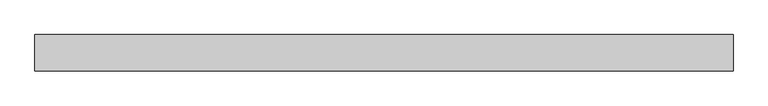
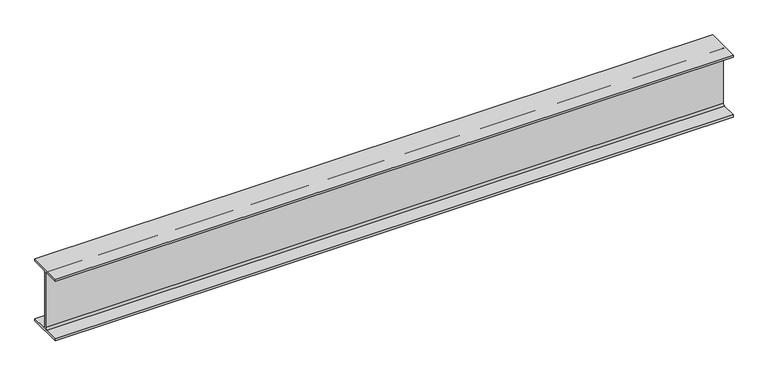
"""IFC4 building model written with IfcOpenShell, lengths in millimetres: beam geometry, Steel Beam_H-KSD3502 : H_SB_ASB_H-250x125x6x9."""

import ifcopenshell
import ifcopenshell.guid

model = None  # the IFC model being written
_history = None  # IfcOwnerHistory: only IFC2X3 demands one
_inside = {}  # id of a spatial element -> (the spatial element, [elements in it])
_under = {}  # id of a project, library or spatial element -> (it, [spatial elements below it])
_declared = {}  # id of a project -> (the project, [libraries it declares])
_typed = {}  # id of a type object -> (the type object, [elements of that type])
_made_of = {}  # id of a material, layer set ... -> (it, [elements and type objects made of it])


def new_model(schema):
    """Start an empty IFC model of exactly this schema.

    Asked for "IFC4X3", IfcOpenShell would pick the latest addendum, in which some entities
    have other attributes; the version numbers below select the first issue.
    IFC2X3 requires an IfcOwnerHistory on every rooted entity: one is made here for all.
    """
    global model, _history
    if schema == "IFC4X3":
        model = ifcopenshell.file(schema_version=(4, 3, 0, 0))
    else:
        model = ifcopenshell.file(schema=schema)
    _inside.clear()
    _under.clear()
    _declared.clear()
    _typed.clear()
    _made_of.clear()
    _history = None
    if model.schema == "IFC2X3":
        org = make("IfcOrganization", Name="unknown")
        user = make(
            "IfcPersonAndOrganization",
            ThePerson=make("IfcPerson", FamilyName="unknown"),
            TheOrganization=org,
        )
        app = make(
            "IfcApplication",
            ApplicationDeveloper=org,
            Version="unknown",
            ApplicationFullName="unknown",
            ApplicationIdentifier="unknown",
        )
        _history = make(
            "IfcOwnerHistory",
            OwningUser=user,
            OwningApplication=app,
            ChangeAction="ADDED",
            CreationDate=0,
        )
    return model


def make(cls, **values):
    """One entity of the class cls with the attributes given. An attribute that is None is left unset."""
    return model.create_entity(
        cls, **{name: value for name, value in values.items() if value is not None}
    )


def rooted(cls, **values):
    """An entity with a GlobalId (a new one), such as an element, a storey or a relation."""
    return make(cls, GlobalId=ifcopenshell.guid.new(), OwnerHistory=_history, **values)


def si_unit(unit_type, name, prefix=None):
    """IfcSIUnit, for example si_unit("LENGTHUNIT", "METRE", prefix="MILLI")."""
    return make("IfcSIUnit", UnitType=unit_type, Prefix=prefix, Name=name)


def assignment(units):
    """IfcUnitAssignment: the units of a project."""
    return None if units is None else make("IfcUnitAssignment", Units=units)


def point(xyz):
    """IfcCartesianPoint."""
    return None if xyz is None else make("IfcCartesianPoint", Coordinates=xyz)


def direction(xyz):
    """IfcDirection."""
    return None if xyz is None else make("IfcDirection", DirectionRatios=xyz)


def frame(location, z_axis=None, x_axis=None):
    """IfcAxis2Placement3D, a coordinate frame: its origin and axes. An axis left out is left unset."""
    return make(
        "IfcAxis2Placement3D",
        Location=point(location),
        Axis=direction(z_axis),
        RefDirection=direction(x_axis),
    )


def frame_2d(location, x_axis=None):
    """IfcAxis2Placement2D, a coordinate frame in the plane: its origin and x axis."""
    return make(
        "IfcAxis2Placement2D", Location=point(location), RefDirection=direction(x_axis)
    )


def origin():
    """The frame at (0, 0, 0) with its axes left unset."""
    return frame((0.0, 0.0, 0.0))


def place(relative_to, where):
    """IfcLocalPlacement: puts the frame where relative to a parent placement (None: the world)."""
    return make(
        "IfcLocalPlacement", PlacementRelTo=relative_to, RelativePlacement=where
    )


def context(
    kind, dimensions, precision=None, world=None, true_north=None, identifier=None
):
    """IfcGeometricRepresentationContext, for example the 3D "Model" context."""
    return make(
        "IfcGeometricRepresentationContext",
        ContextIdentifier=identifier,
        ContextType=kind,
        CoordinateSpaceDimension=dimensions,
        Precision=precision,
        WorldCoordinateSystem=world,
        TrueNorth=true_north,
    )


def project(units=None, contexts=None):
    """IfcProject with its units and contexts."""
    return rooted(
        "IfcProject",
        Name="project",
        RepresentationContexts=contexts,
        UnitsInContext=assignment(units),
    )


def spatial(cls, under=None, at=None, **own):
    """A site, building, storey or space (cls), placed at a placement, below another one or the project."""
    s = rooted(cls, ObjectPlacement=at, **own)
    if under is not None:
        _under.setdefault(under.id(), (under, []))[1].append(s)
    return s


def polyline(points):
    """IfcPolyline through the points."""
    return make("IfcPolyline", Points=[point(p) for p in points])


def circle_curve(where, radius):
    """IfcCircle in the frame where."""
    return make("IfcCircle", Position=where, Radius=radius)


def trimmed(basis, trim1, trim2, sense, master):
    """IfcTrimmedCurve: the piece of a basis curve between two trims."""
    return make(
        "IfcTrimmedCurve",
        BasisCurve=basis,
        Trim1=trim1,
        Trim2=trim2,
        SenseAgreement=sense,
        MasterRepresentation=master,
    )


def segment(curve, same_sense, transition):
    """IfcCompositeCurveSegment."""
    return make(
        "IfcCompositeCurveSegment",
        Transition=transition,
        SameSense=same_sense,
        ParentCurve=curve,
    )


def composite_curve(segments, self_intersect=None):
    """IfcCompositeCurve: segments joined end to end."""
    return make("IfcCompositeCurve", Segments=segments, SelfIntersect=self_intersect)


def outline(outer, holes=None, kind="AREA"):
    """IfcArbitraryClosedProfileDef: a profile drawn as a closed curve; with holes, ...WithVoids."""
    if holes is None:
        return make("IfcArbitraryClosedProfileDef", ProfileType=kind, OuterCurve=outer)
    return make(
        "IfcArbitraryProfileDefWithVoids",
        ProfileType=kind,
        OuterCurve=outer,
        InnerCurves=holes,
    )


def extrude(swept, where, along, depth):
    """IfcExtrudedAreaSolid: the profile swept, set in the frame where, extruded along a direction by depth."""
    return make(
        "IfcExtrudedAreaSolid",
        SweptArea=swept,
        Position=where,
        ExtrudedDirection=direction(along),
        Depth=depth,
    )


def shape(context_of_items, identifier, shape_type, items):
    """IfcShapeRepresentation: the items that make up one representation, for example the "Body"."""
    return make(
        "IfcShapeRepresentation",
        ContextOfItems=context_of_items,
        RepresentationIdentifier=identifier,
        RepresentationType=shape_type,
        Items=items,
    )


def source(mapping_origin, context_of_items, identifier, shape_type, items):
    """IfcRepresentationMap: a shape defined once, which mapped items show again and again."""
    return make(
        "IfcRepresentationMap",
        MappingOrigin=mapping_origin,
        MappedRepresentation=shape(context_of_items, identifier, shape_type, items),
    )


def transform(
    local_origin,
    x_axis=None,
    y_axis=None,
    z_axis=None,
    scale=None,
    scale2=None,
    scale3=None,
    uniform=True,
):
    """IfcCartesianTransformationOperator3D, or its non-uniform kind. x_axis, y_axis, z_axis: its Axis1, 2, 3."""
    if uniform:
        return make(
            "IfcCartesianTransformationOperator3D",
            Axis1=direction(x_axis),
            Axis2=direction(y_axis),
            LocalOrigin=point(local_origin),
            Scale=scale,
            Axis3=direction(z_axis),
        )
    return make(
        "IfcCartesianTransformationOperator3DnonUniform",
        Axis1=direction(x_axis),
        Axis2=direction(y_axis),
        LocalOrigin=point(local_origin),
        Scale=scale,
        Axis3=direction(z_axis),
        Scale2=scale2,
        Scale3=scale3,
    )


def mapped(mapping_source, mapping_target):
    """IfcMappedItem: shows the shape of a source again, moved by a transform."""
    return make(
        "IfcMappedItem", MappingSource=mapping_source, MappingTarget=mapping_target
    )


def made_of(thing, what):
    """Note that an element or type object is made of a material, layer set ...; save() writes the relation."""
    if what is not None:
        _made_of.setdefault(what.id(), (what, []))[1].append(thing)
    return thing


def element(
    cls,
    number,
    at=None,
    inside=None,
    cuts=None,
    type_object=None,
    material=None,
    context=None,
    identifier="Body",
    shape_type=None,
    held_by="IfcProductDefinitionShape",
    body=None,
    shapes=None,
    **own,
):
    """One element of the class cls, such as IfcWall. Its Tag is "e" and its number.

    at: its placement. inside: the storey or other place that contains it. cuts: it is an
    opening in that element (IfcRelVoidsElement). A single representation is given by context,
    identifier, shape_type and body (its items); several are given by shapes. held_by: the class
    of the entity that holds the representations. save() writes the other relations.
    """
    e = rooted(cls, Tag="e%d" % number, ObjectPlacement=at, **own)
    if body is not None:
        shapes = [shape(context, identifier, shape_type, body)]
    if shapes is not None:
        e.Representation = make(held_by, Representations=shapes)
    if inside is not None:
        _inside.setdefault(inside.id(), (inside, []))[1].append(e)
    if cuts is not None:
        rooted(
            "IfcRelVoidsElement", RelatingBuildingElement=cuts, RelatedOpeningElement=e
        )
    if type_object is not None:
        _typed.setdefault(type_object.id(), (type_object, []))[1].append(e)
    return made_of(e, material)


def aggregate(whole, parts):
    """IfcRelAggregates: a whole, such as a stair, and the parts it consists of."""
    return rooted("IfcRelAggregates", RelatingObject=whole, RelatedObjects=parts)


def save(model, path):
    """Write the relations noted so far, then the file.

    IfcRelAggregates (storeys below a building ...), IfcRelContainedInSpatialStructure (elements
    in a storey), IfcRelDefinesByType, IfcRelAssociatesMaterial and IfcRelDeclares: one each for
    every whole, place, type object, material and project.
    """
    for whole, parts in _under.values():
        aggregate(whole, parts)
    for where, things in _inside.values():
        rooted(
            "IfcRelContainedInSpatialStructure",
            RelatedElements=things,
            RelatingStructure=where,
        )
    for kind, things in _typed.values():
        rooted("IfcRelDefinesByType", RelatedObjects=things, RelatingType=kind)
    for what, things in _made_of.values():
        rooted("IfcRelAssociatesMaterial", RelatedObjects=things, RelatingMaterial=what)
    for by, libraries in _declared.values():
        rooted("IfcRelDeclares", RelatingContext=by, RelatedDefinitions=libraries)
    model.write(path)


def beam_c4c65e90(model_context):
    return source(origin(), model_context, "Body", "SweptSolid", [
        extrude(outline(composite_curve([segment(polyline([(82.5, -141.5), (82.5, -151.7), (-82.5, -151.7), (-82.5, -141.5), (-11.9, -141.5)]), True, "CONTINUOUS"), segment(trimmed(circle_curve(frame_2d((-11.9, -132.6)), 8.9), [point((-11.9, -141.5))], [point((-3.0, -132.6))], True, "CARTESIAN"), True, "CONTINUOUS"), segment(polyline([(-3.0, -132.6), (-3.0, 132.6)]), True, "CONTINUOUS"), segment(trimmed(circle_curve(frame_2d((-11.9, 132.6)), 8.9), [point((-3.0, 132.6))], [point((-11.9, 141.5))], True, "CARTESIAN"), True, "CONTINUOUS"), segment(polyline([(-11.9, 141.5), (-82.5, 141.5), (-82.5, 151.7), (82.5, 151.7), (82.5, 141.5), (11.9, 141.5)]), True, "CONTINUOUS"), segment(trimmed(circle_curve(frame_2d((11.9, 132.6)), 8.9), [point((11.9, 141.5))], [point((3.0, 132.6))], True, "CARTESIAN"), True, "CONTINUOUS"), segment(polyline([(3.0, 132.6), (3.0, -132.6)]), True, "CONTINUOUS"), segment(trimmed(circle_curve(frame_2d((11.9, -132.6)), 8.9), [point((3.0, -132.6))], [point((11.9, -141.5))], True, "CARTESIAN"), True, "CONTINUOUS"), segment(polyline([(11.9, -141.5), (82.5, -141.5)]), True, "CONTINUOUS")], self_intersect=False)), frame((-1494.5360727, 0.0, 0.0), z_axis=(1.0, 0.0, 0.0), x_axis=(0.0, 1.0, 0.0)), (0.0, 0.0, 1.0), 3149.3360727),
    ])


if __name__ == "__main__":
    model = new_model("IFC4")
    model_context = context("Model", 3, world=origin())
    ifc_project = project(units=[si_unit("LENGTHUNIT", "METRE", prefix="MILLI")], contexts=[model_context])
    site = spatial("IfcSite", under=ifc_project)
    building = spatial("IfcBuilding", under=site)
    placement = place(None, origin())
    beam_shape = beam_c4c65e90(model_context)
    element("IfcBeam", 1, ObjectType="Steel Beam_H-KSD3502 : H_SB_ASB_H-250x125x6x9", at=placement, inside=building, context=model_context, shape_type="MappedRepresentation", body=[
        mapped(beam_shape, transform((0.0, 0.0, 0.0), x_axis=(1.0, 0.0, 0.0), y_axis=(0.0, 1.0, 0.0), z_axis=(0.0, 0.0, 1.0))),
    ])
    save(model, "model.ifc")

# Revit data of these elements
# Type "Steel Beam_H-KSD3502 : H_SB_ASB_H-250x125x6x9"
#   Width = 12.5 cm
#   Web Thickness = 0.6 cm
#   Web Fillet = 1.2 cm
#   Warping Constant = 42539.8 cm⁶
#   Torsional Moment of Inertia = 7.8102 cm⁴
#   Torsional Modulus = 1.0 cm³
#   Section Area = 37.66 cm²
#   Plastic Modulus weak axis = 73.1 cm³
#   Plastic Modulus strong axis = 366.0 cm³
#   Perimeter = 0.97 m²/m
#   Nominal Weight = 29.60 kgf/m
#   Moment of Inertia weak axis = 294.00 cm⁴
#   Moment of Inertia strong axis = 4050.00 cm⁴
#   Height = 25.0 cm
#   Flange Thickness = 0.9 cm
#   Elastic Modulus weak axis = 47.0 cm³
#   Elastic Modulus strong axis = 324.0 cm³
#   Centroid Vertical = 12.5 cm
#   Centroid Horizontal = 6.25 cm
#   Length [instance default] = 1.5240 m
#   Structural Material [instance default] = Steel, 45-345
#   Assembly Code = ""
# Element 1 (IfcBeam, "Steel Beam_H-KSD3502 : H_SB_ASB_H-250x125x6x9")
#   Structural Material = none
# Materials
#   "Steel, 45-345": class "Metal", colour RGB 189 187 185, transparency 0, Description = "Steel 345 MPa", Cost = 0
